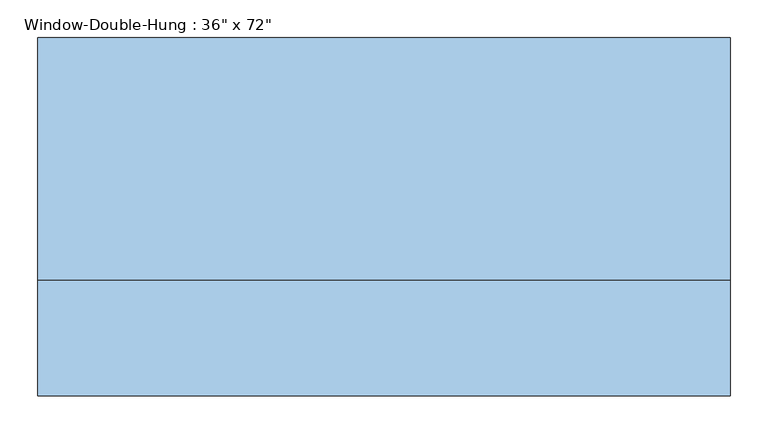
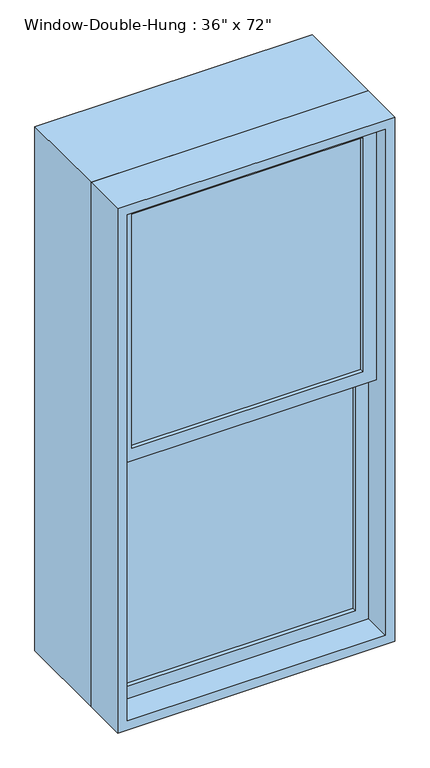
"""IFC4 building model written with IfcOpenShell, lengths in millimetres: window geometry."""

from ifc_helpers import new_model, si_unit, frame, origin, place, context, project, spatial, polyline, outline, extrude, source, transform, mapped, element, save


def window_19547fdf(model_context):
    return source(origin(), model_context, "Body", "SweptSolid", [
        extrude(outline(polyline([(381.0, -138.1125), (-381.0, -138.1125), (-381.0, -131.7625), (381.0, -131.7625), (381.0, -138.1125)])), frame((0.0, 0.0, 990.6), z_axis=(0.0, 0.0, 1.0), x_axis=(1.0, 0.0, 0.0)), (0.0, 0.0, 1.0), 815.975),
        extrude(outline(polyline([(-381.0, -125.4125), (-381.0, -119.0625), (381.0, -119.0625), (381.0, -125.4125), (-381.0, -125.4125)])), frame((0.0, 0.0, 990.6), z_axis=(0.0, 0.0, 1.0), x_axis=(1.0, 0.0, 0.0)), (0.0, 0.0, 1.0), 815.975),
        extrude(outline(polyline([(381.0, -182.5625), (-381.0, -182.5625), (-381.0, -176.2125), (381.0, -176.2125), (381.0, -182.5625)])), frame((0.0, 0.0, 1851.025), z_axis=(0.0, 0.0, 1.0), x_axis=(1.0, 0.0, 0.0)), (0.0, 0.0, 1.0), 815.975),
        extrude(outline(polyline([(-381.0, -169.8625), (-381.0, -163.5125), (381.0, -163.5125), (381.0, -169.8625), (-381.0, -169.8625)])), frame((0.0, 0.0, 1851.025), z_axis=(0.0, 0.0, 1.0), x_axis=(1.0, 0.0, 0.0)), (0.0, 0.0, 1.0), 815.975),
        extrude(outline(polyline([(1851.025, 425.45), (1851.025, -425.45), (946.15, -425.45), (946.15, 425.45), (1851.025, 425.45)]), holes=[polyline([(1806.575, -381.0), (1806.575, 381.0), (990.6, 381.0), (990.6, -381.0), (1806.575, -381.0)])]), frame((0.0, -150.8125, 0.0), z_axis=(0.0, 1.0, 0.0), x_axis=(0.0, 0.0, 1.0)), (0.0, 0.0, 1.0), 44.45),
        extrude(outline(polyline([(2711.45, 425.45), (2711.45, -425.45), (1806.575, -425.45), (1806.575, 425.45), (2711.45, 425.45)]), holes=[polyline([(2667.0, -381.0), (2667.0, 381.0), (1851.025, 381.0), (1851.025, -381.0), (2667.0, -381.0)])]), frame((0.0, -195.2625, 0.0), z_axis=(0.0, 1.0, 0.0), x_axis=(0.0, 0.0, 1.0)), (0.0, 0.0, 1.0), 44.45),
        extrude(outline(polyline([(2743.2, 457.2), (2743.2, -457.2), (914.4, -457.2), (914.4, 457.2), (2743.2, 457.2)]), holes=[polyline([(2711.45, -425.45), (2711.45, 425.45), (946.15, 425.45), (946.15, -425.45), (2711.45, -425.45)])]), frame((0.0, -246.0625, 0.0), z_axis=(0.0, 1.0, 0.0), x_axis=(0.0, 0.0, 1.0)), (0.0, 0.0, 1.0), 152.4),
        extrude(outline(polyline([(2743.2, 457.2), (2743.2, -457.2), (914.4, -457.2), (914.4, 457.2), (2743.2, 457.2)]), holes=[polyline([(2724.15, 438.15), (933.45, 438.15), (933.45, -438.15), (2724.15, -438.15), (2724.15, 438.15)])]), frame((0.0, -93.6625, 0.0), z_axis=(0.0, 1.0, 0.0), x_axis=(0.0, 0.0, 1.0)), (0.0, 0.0, 1.0), 320.675),
    ])


if __name__ == "__main__":
    model = new_model("IFC4")
    model_context = context("Model", 3, world=origin())
    ifc_project = project(units=[si_unit("LENGTHUNIT", "METRE", prefix="MILLI")], contexts=[model_context])
    site = spatial("IfcSite", under=ifc_project)
    building = spatial("IfcBuilding", under=site)
    placement = place(None, origin())
    window_shape = window_19547fdf(model_context)
    element("IfcWindow", 1, ObjectType="Window-Double-Hung : 36\" x 72\"", at=placement, inside=building, context=model_context, shape_type="MappedRepresentation", body=[
        mapped(window_shape, transform((0.0, 0.0, 0.0), x_axis=(1.0, 0.0, 0.0), y_axis=(0.0, 1.0, 0.0), z_axis=(0.0, 0.0, 1.0))),
    ])
    save(model, "model.ifc")

# Revit data of these elements
# Type "Window-Double-Hung : 36\" x 72\""
#   Type Mark = "22"
#   Fire Rating = "0.5h"
#   Construction Type Id = "DG-DR"
#   Assembly Code = "B2020100"
#   Analytic Construction = "Double glazing - domestic"
#   Wall Thickness [instance default] = 0' - 6"
#   Visual Light Transmittance = 0.81
#   Thermal Resistance (R) = 1.8146 (h·ft²·°F)/BTU
#   Solar Heat Gain Coefficient = 0.76
#   Rough Width = 3' - 0 1/2"
#   Rough Height = 6' - 0 1/2"
#   Muntin Width = 2' - 6"
#   Muntin Height = 2' - 8 1/8"
#   Interior Wall Closure [instance default] = 0' - 1 1/2"
#   Heat Transfer Coefficient (U) = 0.5511 BTU/(h·ft²·°F)
#   Frame Extension [instance default] = 0' - 2"
#   Exterior Wall Closure [instance default] = 0' - 0 1/2"
#   Extension Jamb [instance default] = 0' - 0 3/4"
#   Height = 6' - 0"
#   Width = 3' - 0"
#   Window Inset [instance default] = 0' - 0 3/4"
#   Top Muntin Visibility = yes
#   Interior Trim Visibility [instance default] = yes
#   Indicator Visibility [instance default] = yes
#   Exterior Trim Visibility [instance default] = yes
#   Extension Jamb Visibility [instance default] = yes
#   Define Thermal Properties by = 1
#   Bottom Muntin Visibility = yes
#   Muntin Pattern = Muntin Pattern_2x2 : Muntin Pattern_2x2
#   Interior Trim Material = Wood - Stained
#   Interior Trim = Trim-Window-Interior-Flat : Picture Frame
#   Interior Frame Material = Wood - Stained
#   Glass Panel Material = Glass
#   Exterior Trim Material = Clad - White
#   Exterior Trim = Trim-Window-Exterior-Flat : with Sill
#   Exterior Frame Material = Clad - White
#   Wall Closure = (empty or 0)
# Element 1 (IfcWindow, "Window-Double-Hung : 36\" x 72\"")
#   Wall Thickness = 1' - 5 7/8"
#   Extension Jamb = 1' - 0 5/8"
#   Materials on its faces: "Wood - Stained", "Glass", "Clad - White"
# Materials
#   "Wood - Stained": class "Wood", colour RGB 224 178 126, transparency 0, Cost = 0
#   "Glass": class "Unassigned", colour RGB 0 128 192, transparency 0.75, Description = "Glass"
#   "Clad - White": class "Wood", colour RGB 242 242 238, transparency 0, Cost = 0
